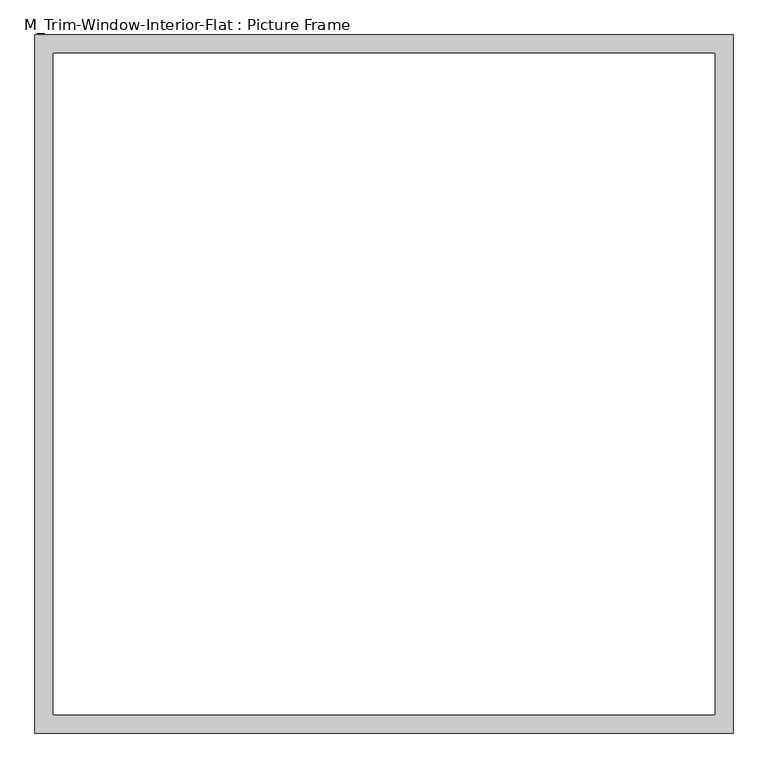
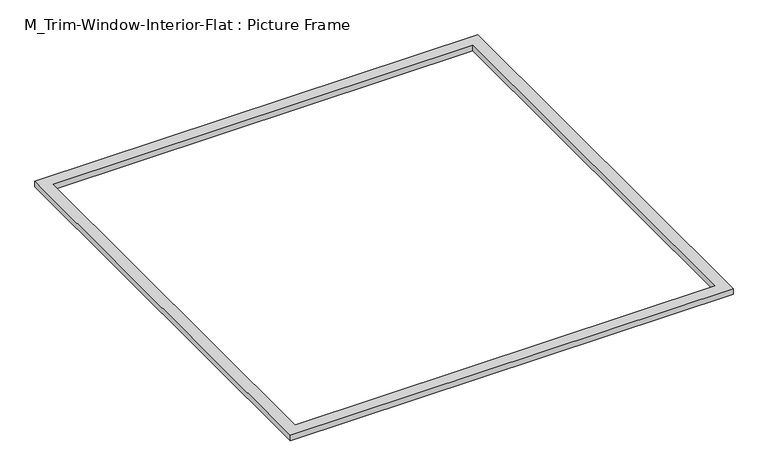
"""IFC4 building model written with IfcOpenShell, lengths in millimetres: proxy geometry, M_Trim-Window-Interior-Flat : Picture Frame."""

from ifc_helpers import new_model, si_unit, origin, origin_with_axes, place, context, project, spatial, polyline, outline, extrude, source, transform, mapped, element, save


def m_trim_window_interior_flat_picture_frame_437a4412(model_context):
    return source(origin(), model_context, "Body", "SweptSolid", [
        extrude(outline(polyline([(1147.3, 47.3), (1147.3, -2247.3), (-1147.3, -2247.3), (-1147.3, 47.3), (1147.3, 47.3)]), holes=[polyline([(1087.3, -12.7), (-1087.3, -12.7), (-1087.3, -2187.3), (1087.3, -2187.3), (1087.3, -12.7)])]), origin_with_axes(), (0.0, 0.0, 1.0), 30.0),
    ])


if __name__ == "__main__":
    model = new_model("IFC4")
    model_context = context("Model", 3, world=origin())
    ifc_project = project(units=[si_unit("LENGTHUNIT", "METRE", prefix="MILLI")], contexts=[model_context])
    site = spatial("IfcSite", under=ifc_project)
    building = spatial("IfcBuilding", under=site)
    placement = place(None, origin())
    m_trim_window_interior_flat_picture_frame_shape = m_trim_window_interior_flat_picture_frame_437a4412(model_context)
    element("IfcBuildingElementProxy", 1, Name="M_Trim-Window-Interior-Flat : Picture Frame", ObjectType="M_Trim-Window-Interior-Flat : Picture Frame", at=placement, inside=building, context=model_context, shape_type="MappedRepresentation", body=[
        mapped(m_trim_window_interior_flat_picture_frame_shape, transform((0.0, 0.0, 0.0), x_axis=(1.0, 0.0, 0.0), y_axis=(0.0, 1.0, 0.0), z_axis=(0.0, 0.0, 1.0))),
    ])
    save(model, "model.ifc")

# Revit data of these elements
# Type "M_Trim-Window-Interior-Flat : Picture Frame"
#   Trim Thickness_Picture Frame = 0.03 m
#   Trim Width = 0.06 m
#   Trim Thickness_with Sill = 0.02 m
#   Sill Thickness = 0.03 m
#   Opening Width [instance default] = 0.60 m
#   Opening Height [instance default] = 0.90 m
#   Default Elevation = 1.20 m
#   Sill = no
#   Picture Frame = yes
#   Trim Material [instance default] = none
# Element 1 (IfcBuildingElementProxy, "M_Trim-Window-Interior-Flat : Picture Frame")
#   Opening Width = 2.20 m
#   Opening Height = 2.20 m
#   Trim Material = Wood - Stained
#   Materials on its faces: "Wood - Stained"
# Materials
#   "Wood - Stained": class "Wood", colour RGB 227 170 128, transparency 0, Cost = 0
